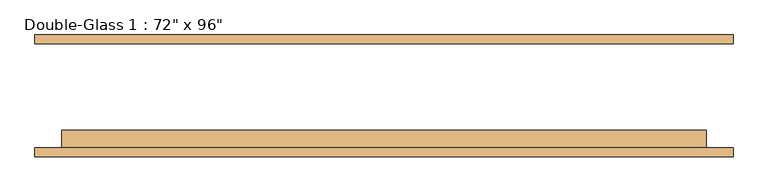
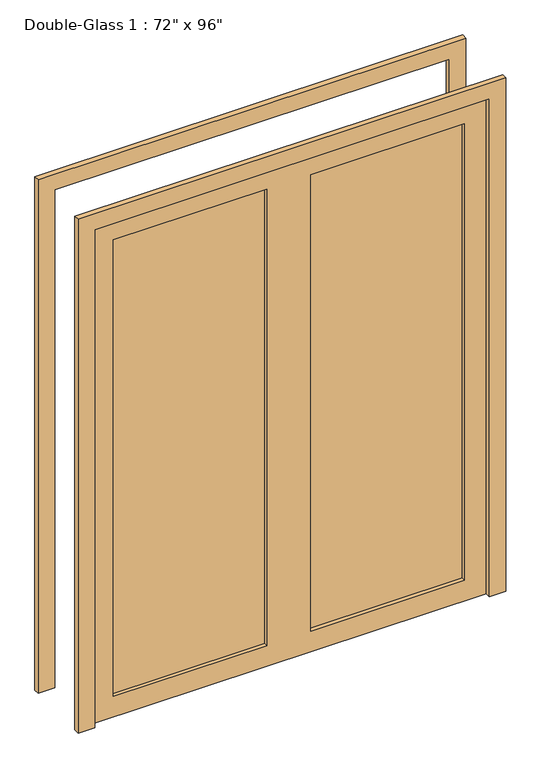
"""IFC4 building model written with IfcOpenShell, lengths in millimetres: door geometry."""

from ifc_helpers import new_model, si_unit, frame, origin, place, context, project, spatial, polyline, outline, extrude, source, transform, mapped, element, save


def door_42bba6ff(model_context):
    return source(origin(), model_context, "Body", "SweptSolid", [
        extrude(outline(polyline([(0.0, 990.6), (2514.6, 990.6), (2514.6, -990.6), (0.0, -990.6), (0.0, -914.4), (2438.4, -914.4), (2438.4, 914.4), (0.0, 914.4), (0.0, 990.6)])), frame((0.0, 145.25625, 0.0), z_axis=(0.0, 1.0, 0.0), x_axis=(0.0, 0.0, 1.0)), (0.0, 0.0, 1.0), 25.4),
        extrude(outline(polyline([(2438.4, 914.4), (0.0, 914.4), (0.0, 990.6), (2514.6, 990.6), (2514.6, -990.6), (0.0, -990.6), (0.0, -914.4), (2438.4, -914.4), (2438.4, 914.4)])), frame((0.0, -175.41875, 0.0), z_axis=(0.0, 1.0, 0.0), x_axis=(0.0, 0.0, 1.0)), (0.0, 0.0, 1.0), 25.4),
        extrude(outline(polyline([(812.8, -124.61875), (812.8, -131.7625), (101.6, -131.7625), (101.6, -124.61875), (812.8, -124.61875)])), frame((0.0, 0.0, 101.6), z_axis=(0.0, 0.0, 1.0), x_axis=(1.0, 0.0, 0.0)), (0.0, 0.0, 1.0), 2235.2),
        extrude(outline(polyline([(-101.6, -124.61875), (-101.6, -131.7625), (-812.8, -131.7625), (-812.8, -124.61875), (-101.6, -124.61875)])), frame((0.0, 0.0, 101.6), z_axis=(0.0, 0.0, 1.0), x_axis=(1.0, 0.0, 0.0)), (0.0, 0.0, 1.0), 2235.2),
        extrude(outline(polyline([(2438.4, 914.4), (2438.4, -914.4), (0.0, -914.4), (0.0, 914.4), (2438.4, 914.4)]), holes=[polyline([(2336.8, -101.6), (101.6, -101.6), (101.6, -812.8), (2336.8, -812.8), (2336.8, -101.6)]), polyline([(2336.8, 812.8), (101.6, 812.8), (101.6, 101.6), (2336.8, 101.6), (2336.8, 812.8)])]), frame((0.0, -150.01875, 0.0), z_axis=(0.0, 1.0, 0.0), x_axis=(0.0, 0.0, 1.0)), (0.0, 0.0, 1.0), 50.8),
    ])


if __name__ == "__main__":
    model = new_model("IFC4")
    model_context = context("Model", 3, world=origin())
    ifc_project = project(units=[si_unit("LENGTHUNIT", "METRE", prefix="MILLI")], contexts=[model_context])
    site = spatial("IfcSite", under=ifc_project)
    building = spatial("IfcBuilding", under=site)
    placement = place(None, origin())
    door_shape = door_42bba6ff(model_context)
    element("IfcDoor", 1, ObjectType="Double-Glass 1 : 72\" x 96\"", at=placement, inside=building, context=model_context, shape_type="MappedRepresentation", body=[
        mapped(door_shape, transform((0.0, 0.0, 0.0), x_axis=(1.0, 0.0, 0.0), y_axis=(0.0, 1.0, 0.0), z_axis=(0.0, 0.0, 1.0))),
    ])
    save(model, "model.ifc")

# Revit data of these elements
# Type "Double-Glass 1 : 72\" x 96\""
#   Type Mark = "30"
#   Construction Type Id = "MDOOR"
#   Assembly Code = "C1020"
#   Analytic Construction = "Metal"
#   Thickness = 0' - 2"
#   Thermal Resistance (R) = 0.270118 (m²·K)/W
#   Heat Transfer Coefficient (U) = 3.70223 W/(m²·K)
#   Height = 8' - 0"
#   Rail Width - Base = 0' - 4"
#   Rail Width - Top = 0' - 4"
#   Stile Width - Hinge = 0' - 4"
#   Stile Width - Latch = 0' - 4"
#   Trim Projection = 0' - 1"
#   Trim Width = 0' - 3"
#   Width = 6' - 0"
#   Door Material = Aluminum
#   Frame Material = Aluminum
#   Visual Light Transmittance = 0
#   Solar Heat Gain Coefficient = 0
#   Function = (empty or 0)
#   Wall Closure = (empty or 0)
# Element 1 (IfcDoor, "Double-Glass 1 : 72\" x 96\"")
#   Materials on its faces: "Aluminum", "Glass"
# Materials
#   "Aluminum": class "Metal", colour RGB 247 247 247, transparency 0, Description = "Aluminum 6061", Cost = 0
#   "Glass": class "Glass", colour RGB 0 128 192, transparency 0.75, Description = "Soda Lime Glass", Cost = 0
